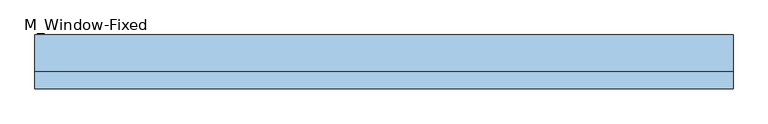
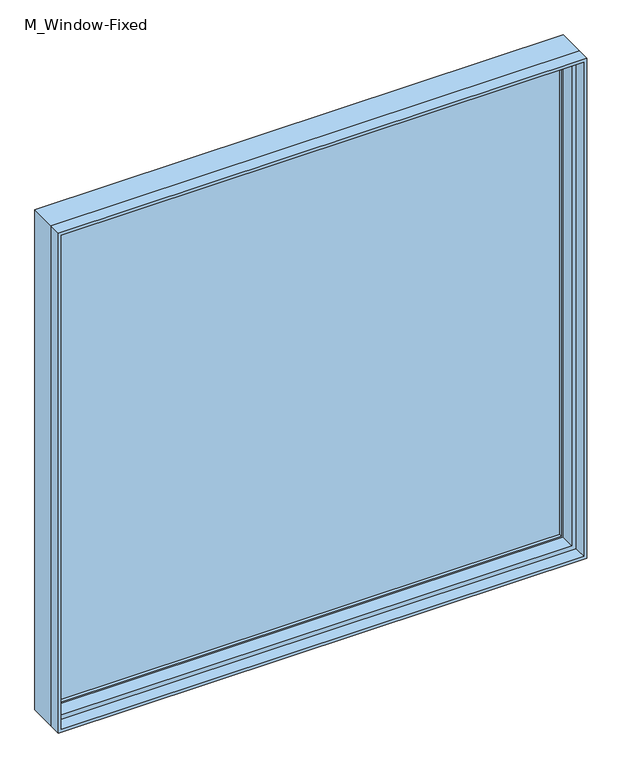
"""IFC4 building model written with IfcOpenShell, lengths in millimetres: window geometry, M_Window-Fixed : 2200 x 2200mm DAPC."""

from ifc_helpers import new_model, si_unit, frame, origin, place, context, project, spatial, polyline, outline, extrude, faceted_brep, source, transform, mapped, element, save


def m_window_fixed_1fa8549e(model_context):
    return source(origin(), model_context, "Body", "SolidModel", [
        faceted_brep([(1100.0, -20.25, 3100.0), (1100.0, 94.05, 3100.0), (-1100.0, 94.05, 3100.0), (-1100.0, -20.25, 3100.0), (-1100.0, 94.05, 900.0), (-1100.0, -20.25, 900.0), (1100.0, 94.05, 900.0), (1100.0, -20.25, 900.0), (1068.25, -20.25, 3068.25), (1068.25, -20.25, 931.75), (-1068.25, -20.25, 931.75), (-1068.25, -20.25, 3068.25), (-1087.3, 94.05, 3087.3), (-1087.3, 94.05, 912.7), (1087.3, 94.05, 912.7), (1087.3, 94.05, 3087.3), (1068.25, 43.25, 3068.25), (-1068.25, 43.25, 3068.25), (1087.3, 43.25, 3087.3), (-1087.3, 43.25, 3087.3), (-1068.25, 43.25, 931.75), (-1087.3, 43.25, 912.7), (1068.25, 43.25, 931.75), (1087.3, 43.25, 912.7)], [[[0, 1, 2, 3]], [[3, 2, 4, 5]], [[5, 4, 6, 7]], [[3, 5, 7, 0], [8, 9, 10, 11]], [[7, 6, 1, 0]], [[1, 6, 4, 2], [12, 13, 14, 15]], [[16, 8, 11, 17]], [[15, 18, 19, 12]], [[17, 11, 10, 20]], [[12, 19, 21, 13]], [[20, 10, 9, 22]], [[13, 21, 23, 14]], [[22, 9, 8, 16]], [[18, 23, 21, 19], [17, 20, 22, 16]], [[14, 23, 18, 15]]]),
        extrude(outline(polyline([(3100.0, -1100.0), (900.0, -1100.0), (900.0, 1100.0), (3100.0, 1100.0), (3100.0, -1100.0)]), holes=[polyline([(3087.3, 1087.3), (912.7, 1087.3), (912.7, -1087.3), (3087.3, -1087.3), (3087.3, 1087.3)])]), frame((0.0, -75.0, 0.0), z_axis=(0.0, 1.0, 0.0), x_axis=(0.0, 0.0, 1.0)), (0.0, 0.0, 1.0), 54.75),
        extrude(outline(polyline([(912.7, 1087.3), (3087.3, 1087.3), (3087.3, -1087.3), (912.7, -1087.3), (912.7, 1087.3)]), holes=[polyline([(938.1, -1061.9), (3061.9, -1061.9), (3061.9, 1061.9), (938.1, 1061.9), (938.1, -1061.9)])]), frame((0.0, 43.25, 0.0), z_axis=(0.0, 1.0, 0.0), x_axis=(0.0, 0.0, 1.0)), (0.0, 0.0, 1.0), 44.45),
        extrude(outline(polyline([(1061.9, 75.0), (1061.9, 68.65), (-1061.9, 68.65), (-1061.9, 75.0), (1061.9, 75.0)])), frame((0.0, 0.0, 938.1), z_axis=(0.0, 0.0, 1.0), x_axis=(1.0, 0.0, 0.0)), (0.0, 0.0, 1.0), 2123.8),
        extrude(outline(polyline([(-1061.9, 55.95), (-1061.9, 62.3), (1061.9, 62.3), (1061.9, 55.95), (-1061.9, 55.95)])), frame((0.0, 0.0, 938.1), z_axis=(0.0, 0.0, 1.0), x_axis=(1.0, 0.0, 0.0)), (0.0, 0.0, 1.0), 2123.8),
    ])


if __name__ == "__main__":
    model = new_model("IFC4")
    model_context = context("Model", 3, world=origin())
    ifc_project = project(units=[si_unit("LENGTHUNIT", "METRE", prefix="MILLI")], contexts=[model_context])
    site = spatial("IfcSite", under=ifc_project)
    building = spatial("IfcBuilding", under=site)
    placement = place(None, origin())
    m_window_fixed_shape = m_window_fixed_1fa8549e(model_context)
    element("IfcWindow", 1, ObjectType="M_Window-Fixed : 2200 x 2200mm DAPC", at=placement, inside=building, context=model_context, shape_type="MappedRepresentation", body=[
        mapped(m_window_fixed_shape, transform((0.0, 0.0, 0.0), x_axis=(1.0, 0.0, 0.0), y_axis=(0.0, 1.0, 0.0), z_axis=(0.0, 0.0, 1.0))),
    ])
    save(model, "model.ifc")

# Revit data of these elements
# Type "M_Window-Fixed : 2200 x 2200mm DAPC"
#   Type Mark = "40"
#   Fire Rating = "0.5h"
#   Analytic Construction = "Double glazing - domestic"
#   Window Inset [instance default] = 0.00 m
#   Wall Thickness [instance default] = 0.15 m
#   Visual Light Transmittance = 0.81
#   Thermal Resistance (R) = 0.319569 (m²·K)/W
#   Solar Heat Gain Coefficient = 0.76
#   Rough Width = 2.215 m
#   Rough Height = 2.215 m
#   Interior Wall Closure [instance default] = 0.05475 m
#   Height = 2.20 m
#   Heat Transfer Coefficient (U) = 3.12929 W/(m²·K)
#   Frame Extension [instance default] = 0.00635 m
#   Exterior Wall Closure [instance default] = 0.03175 m
#   Extension Jamb [instance default] = 0.05475 m
#   Default Sill Height = 0.90 m
#   Width = 2.20 m
#   Muntin Visibility = yes
#   Interior Trim Visibility [instance default] = yes
#   Exterior Trim Visibility [instance default] = yes
#   Extension Jamb Visibility [instance default] = yes
#   Muntin Pattern = M_Muntin Pattern_2x2 : M_Muntin Pattern_2x2
#   Interior Trim Material = Wood - Stained
#   Interior Trim = M_Trim-Window-Interior-Flat : Picture Frame
#   Interior Frame Material = Wood - Stained
#   Glass Panel Material = Glass
#   Exterior Trim Material = Clad - White
#   Exterior Trim = M_Trim-Window-Exterior-Flat : with Sill
#   Exterior Frame Material = Clad - White
#   Wall Closure = (empty or 0)
# Element 1 (IfcWindow, "M_Window-Fixed : 2200 x 2200mm DAPC")
#   Materials on its faces: "Wood - Stained", "Glass", "Clad - White"
# Materials
#   "Wood - Stained": class "Wood", colour RGB 227 170 128, transparency 0, Cost = 0
#   "Glass": class "Glass", colour RGB 0 0 255, transparency 0.75, Description = "Soda Lime Glass", Cost = 0
#   "Clad - White": class "Wood", colour RGB 242 242 238, transparency 0, Cost = 0
